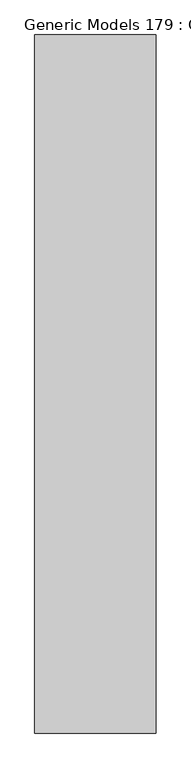
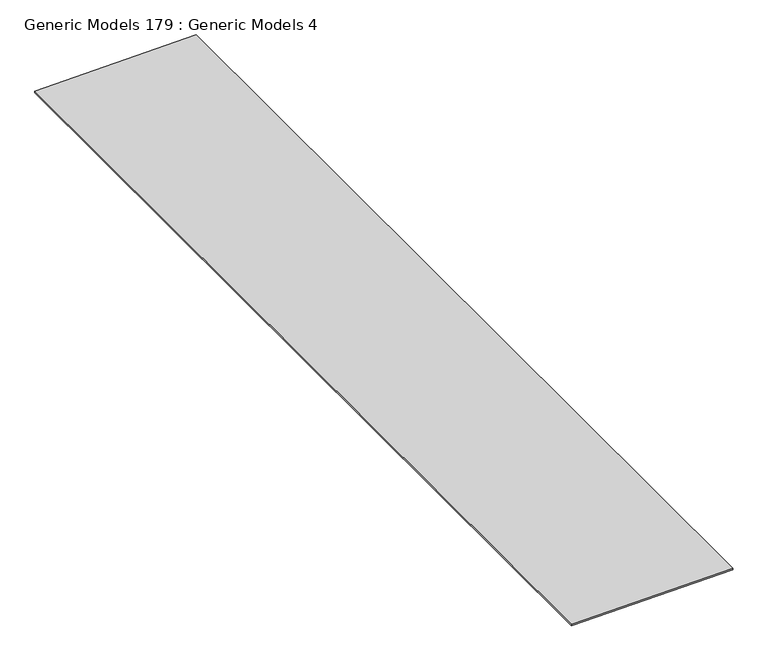
"""IFC4 building model written with IfcOpenShell, lengths in millimetres: proxy geometry, Generic Models 179 : Generic Models 4."""

from ifc_helpers import new_model, si_unit, frame, origin, place, context, project, spatial, polyline, outline, extrude, source, transform, mapped, element, save


def generic_models_179_generic_models_4_49569a4c(model_context):
    return source(origin(), model_context, "Body", "SweptSolid", [
        extrude(outline(polyline([(0.0, -1306.5462675), (0.0, 0.0), (7518.4, 0.0), (7518.4, -1306.5462675), (0.0, -1306.5462675)])), frame((-6618.6468407, -464.1230338, 126712.7660928), z_axis=(-0.017452406437285763, 0.0, 0.9998476951563913), x_axis=(0.0, 1.0, 0.0)), (0.0, 0.0, 1.0), 12.7),
    ])


if __name__ == "__main__":
    model = new_model("IFC4")
    model_context = context("Model", 3, world=origin())
    ifc_project = project(units=[si_unit("LENGTHUNIT", "METRE", prefix="MILLI")], contexts=[model_context])
    site = spatial("IfcSite", under=ifc_project)
    building = spatial("IfcBuilding", under=site)
    placement = place(None, origin())
    generic_models_179_generic_models_4_shape = generic_models_179_generic_models_4_49569a4c(model_context)
    element("IfcBuildingElementProxy", 1, Name="Generic Models 179 : Generic Models 4", ObjectType="Generic Models 179 : Generic Models 4", at=placement, inside=building, context=model_context, shape_type="MappedRepresentation", body=[
        mapped(generic_models_179_generic_models_4_shape, transform((0.0, 0.0, 0.0), x_axis=(1.0, 0.0, 0.0), y_axis=(0.0, 1.0, 0.0), z_axis=(0.0, 0.0, 1.0))),
    ])
    save(model, "model.ifc")

# Revit data of these elements
# Element 1 (IfcBuildingElementProxy, "Generic Models 179 : Generic Models 4")
#   Materials on its faces: "_1/2\" CDX PLYWOOD"
# Materials
#   "_1/2\" CDX PLYWOOD": class "Generic", colour RGB 98 75 74, transparency 0, Cost = 0
